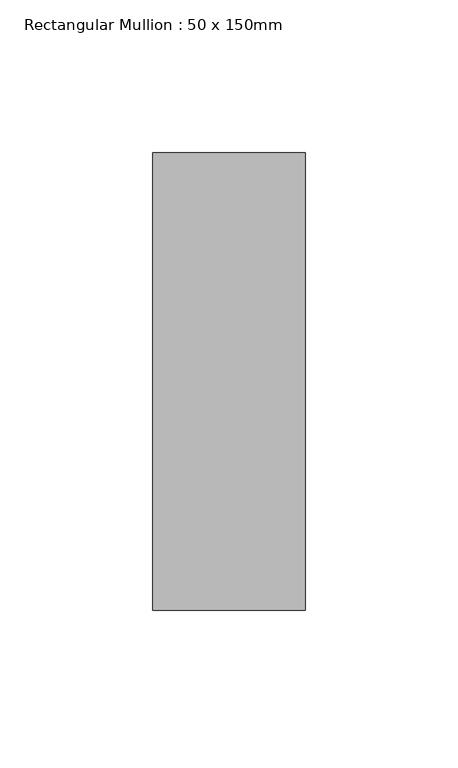
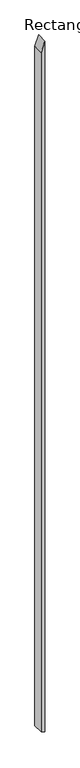
"""IFC4 building model written with IfcOpenShell, lengths in millimetres: member geometry, Rectangular Mullion : 50 x 150mm."""

from ifc_helpers import new_model, si_unit, frame, origin, place, context, project, spatial, polyline, outline, extrude, source, transform, mapped, element, save


def rectangular_mullion_50_x_150mm_36cf8f86(model_context):
    return source(origin(), model_context, "Body", "SweptSolid", [
        extrude(outline(polyline([(0.0, 0.0), (-150.2928962, -50.0), (-10109.8797934, -50.0), (-10126.5139795, 0.0), (0.0, 0.0)])), frame((0.0, -75.0, 0.0), z_axis=(0.0, 1.0, 0.0), x_axis=(0.0, 0.0, 1.0)), (0.0, 0.0, 1.0), 150.0),
    ])


if __name__ == "__main__":
    model = new_model("IFC4")
    model_context = context("Model", 3, world=origin())
    ifc_project = project(units=[si_unit("LENGTHUNIT", "METRE", prefix="MILLI")], contexts=[model_context])
    site = spatial("IfcSite", under=ifc_project)
    building = spatial("IfcBuilding", under=site)
    placement = place(None, origin())
    rectangular_mullion_50_x_150mm_shape = rectangular_mullion_50_x_150mm_36cf8f86(model_context)
    element("IfcMember", 1, ObjectType="Rectangular Mullion : 50 x 150mm", at=placement, inside=building, context=model_context, shape_type="MappedRepresentation", body=[
        mapped(rectangular_mullion_50_x_150mm_shape, transform((0.0, 0.0, 0.0), x_axis=(1.0, 0.0, 0.0), y_axis=(0.0, 1.0, 0.0), z_axis=(0.0, 0.0, 1.0))),
    ])
    save(model, "model.ifc")

# Revit data of these elements
# Type "Rectangular Mullion : 50 x 150mm"
#   built-in parameter 1007304 = 0.492126 (stored number, unit not read)
#   built-in parameter 1007301 = 0.082021 (stored number, unit not read)
#   built-in parameter 1007300 = 0.082021 (stored number, unit not read)
# Element 1 (IfcMember, "Rectangular Mullion : 50 x 150mm")
#   Materials on its faces: "Metal - Aluminium"
# Materials
#   "Metal - Aluminium": class "Metal", colour RGB 247 247 247, transparency 0
